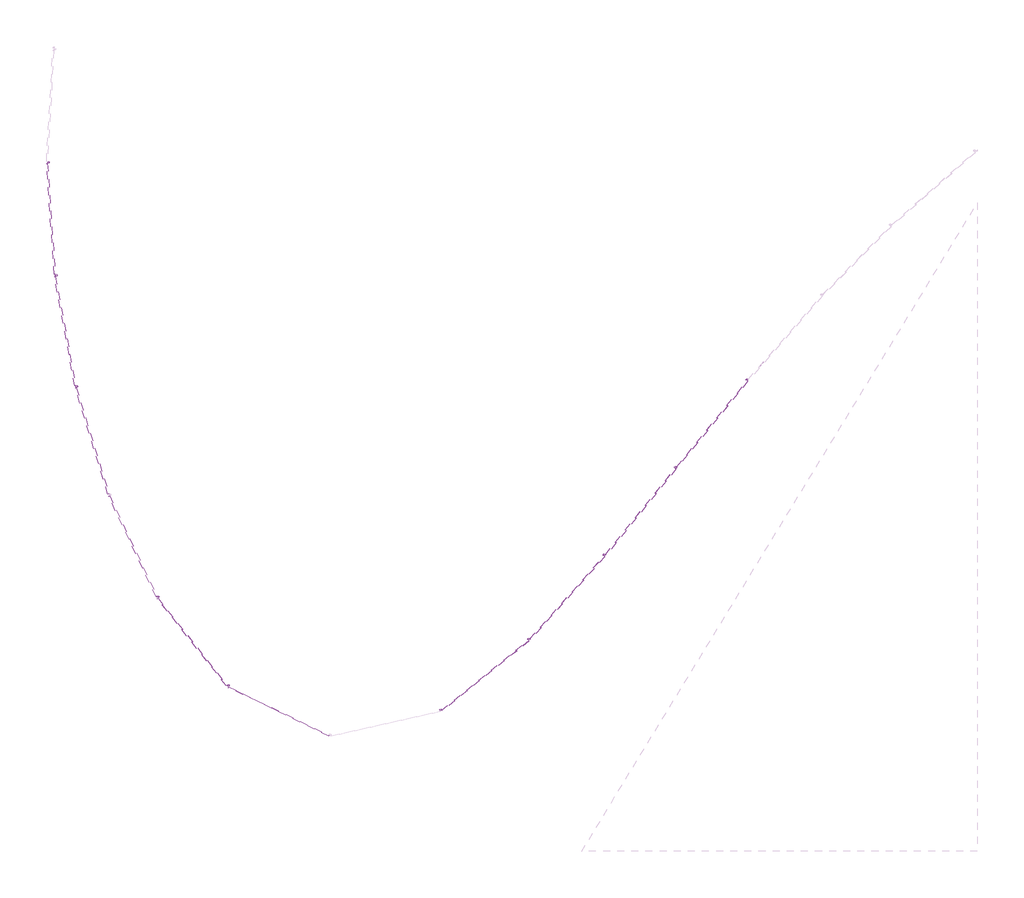
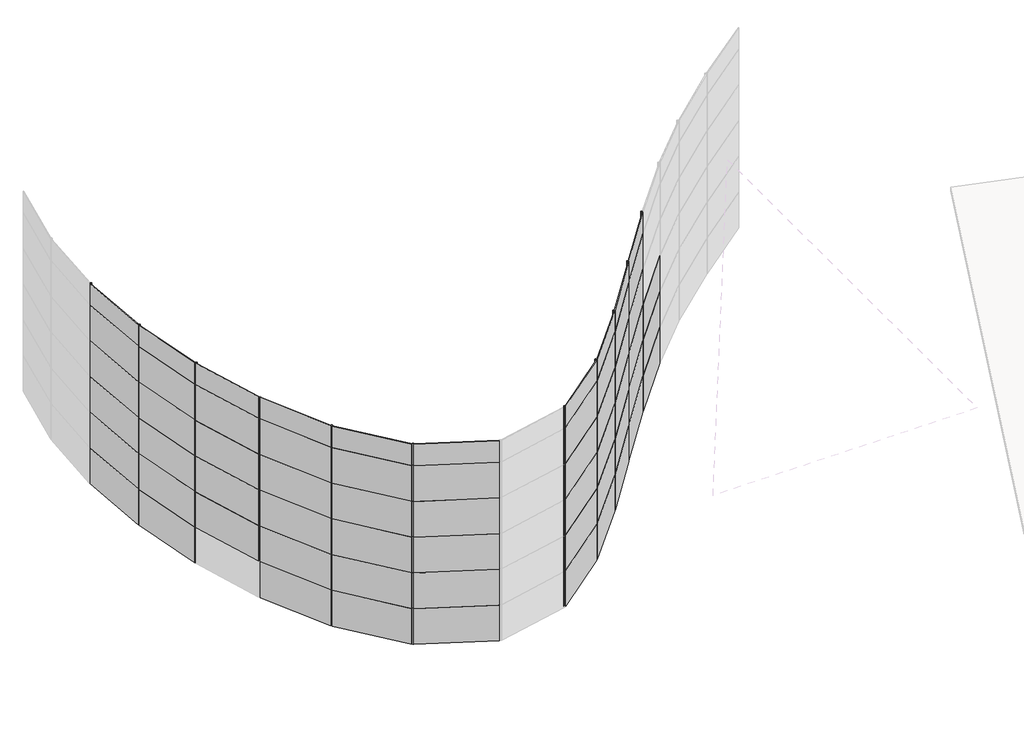
# One storey, part 4 of 8: 62 plates, 60 members.
# Revit data of these elements (continued)
# Type "Montante circular : 25 mm Raio"
#   built-in parameter 1007350 = 0.082021 (stored number, unit not read)
# Type "Painel do sistema : Envidraçado"
#   Construction Type Id = "GSP4R"
#   Analytic Construction = "Vidraça única Pilkington 1/8 pol"
#   Visual Light Transmittance = 0.9
#   Solar Heat Gain Coefficient = 0.86
#   Heat Transfer Coefficient (U) = 6.7069 W/(m²·K)
# Elements 1, 2, 3, 4, 5, 6, 7, 8, 9, 10, 11, 12, 13, 14, 15, 16, 17, 18, 19, 20, 21, 22, 23, 24, 25, 26, 27, 28, 29, 30, 31, 32, 33, 34, 35, 36, 37, 38, 39, 40, 41, 42, 43, 44, 45, 46, 47, 48, 49, 50, 51, 52, 53, 54, 55, 56, 57, 58, 59, 60 (IfcMember, "Montante circular : 25 mm Raio")
#   Phase Created = Construção nova
#   Materials on its faces: "Alumín."
# Elements 61, 62, 63, 64, 65, 66, 67, 68, 69, 70, 71, 72, 73, 74, 75, 76, 77, 78, 79, 80, 81, 82, 83, 84, 85, 86, 87, 88, 89, 90, 91, 92, 93, 94, 95, 96, 97, 98, 99, 100, 101, 102, 103, 104, 105, 106, 107, 108, 109, 110, 111, 112, 113, 114, 115, 116, 117, 118, 119, 120, 121, 122 (IfcPlate, "Painel do sistema : Envidraçado")
#   Phase Created = Construção nova
#   Materials on its faces: "Vidro"
# Materials
#   "Alumín.": class "Metal", colour RGB 247 247 247, transparency 0, Description = "Alumín. 6061", Cost = 0
#   "Vidro": class "Vidro", colour RGB 0 128 192, transparency 0.9, Description = "Vidro de sílica", Cost = 0
